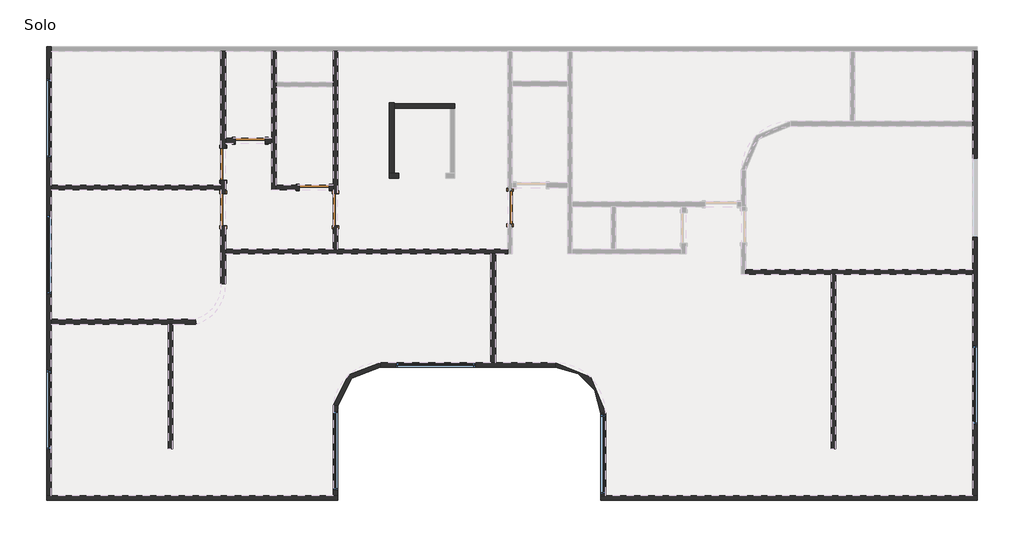
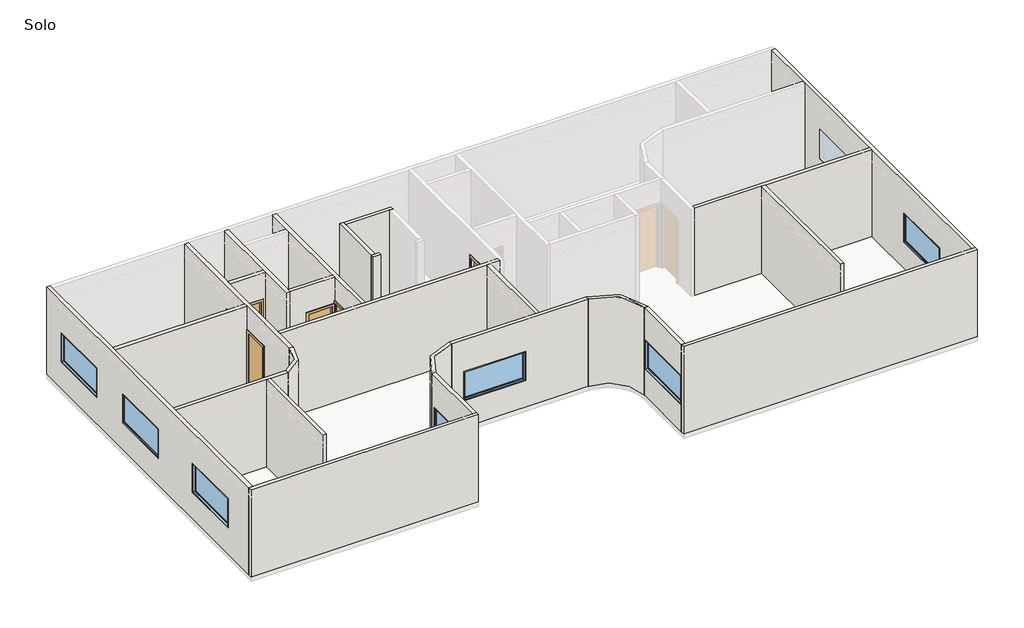
# One storey, part 1 of 2: 25 walls, 7 windows, 6 doors.
"""IFC4 building model written with IfcOpenShell, lengths in millimetres."""

import ifcopenshell
import ifcopenshell.guid

model = None  # the IFC model being written
_history = None  # IfcOwnerHistory: only IFC2X3 demands one
_inside = {}  # id of a spatial element -> (the spatial element, [elements in it])
_under = {}  # id of a project, library or spatial element -> (it, [spatial elements below it])
_declared = {}  # id of a project -> (the project, [libraries it declares])
_typed = {}  # id of a type object -> (the type object, [elements of that type])
_made_of = {}  # id of a material, layer set ... -> (it, [elements and type objects made of it])


def new_model(schema):
    """Start an empty IFC model of exactly this schema.

    Asked for "IFC4X3", IfcOpenShell would pick the latest addendum, in which some entities
    have other attributes; the version numbers below select the first issue.
    IFC2X3 requires an IfcOwnerHistory on every rooted entity: one is made here for all.
    """
    global model, _history
    if schema == "IFC4X3":
        model = ifcopenshell.file(schema_version=(4, 3, 0, 0))
    else:
        model = ifcopenshell.file(schema=schema)
    _inside.clear()
    _under.clear()
    _declared.clear()
    _typed.clear()
    _made_of.clear()
    _history = None
    if model.schema == "IFC2X3":
        org = make("IfcOrganization", Name="unknown")
        user = make(
            "IfcPersonAndOrganization",
            ThePerson=make("IfcPerson", FamilyName="unknown"),
            TheOrganization=org,
        )
        app = make(
            "IfcApplication",
            ApplicationDeveloper=org,
            Version="unknown",
            ApplicationFullName="unknown",
            ApplicationIdentifier="unknown",
        )
        _history = make(
            "IfcOwnerHistory",
            OwningUser=user,
            OwningApplication=app,
            ChangeAction="ADDED",
            CreationDate=0,
        )
    return model


def make(cls, **values):
    """One entity of the class cls with the attributes given. An attribute that is None is left unset."""
    return model.create_entity(
        cls, **{name: value for name, value in values.items() if value is not None}
    )


def rooted(cls, **values):
    """An entity with a GlobalId (a new one), such as an element, a storey or a relation."""
    return make(cls, GlobalId=ifcopenshell.guid.new(), OwnerHistory=_history, **values)


def si_unit(unit_type, name, prefix=None):
    """IfcSIUnit, for example si_unit("LENGTHUNIT", "METRE", prefix="MILLI")."""
    return make("IfcSIUnit", UnitType=unit_type, Prefix=prefix, Name=name)


def assignment(units):
    """IfcUnitAssignment: the units of a project."""
    return None if units is None else make("IfcUnitAssignment", Units=units)


def point(xyz):
    """IfcCartesianPoint."""
    return None if xyz is None else make("IfcCartesianPoint", Coordinates=xyz)


def direction(xyz):
    """IfcDirection."""
    return None if xyz is None else make("IfcDirection", DirectionRatios=xyz)


def frame(location, z_axis=None, x_axis=None):
    """IfcAxis2Placement3D, a coordinate frame: its origin and axes. An axis left out is left unset."""
    return make(
        "IfcAxis2Placement3D",
        Location=point(location),
        Axis=direction(z_axis),
        RefDirection=direction(x_axis),
    )


def frame_2d(location, x_axis=None):
    """IfcAxis2Placement2D, a coordinate frame in the plane: its origin and x axis."""
    return make(
        "IfcAxis2Placement2D", Location=point(location), RefDirection=direction(x_axis)
    )


def origin():
    """The frame at (0, 0, 0) with its axes left unset."""
    return frame((0.0, 0.0, 0.0))


def origin_with_axes():
    """The frame at (0, 0, 0) with the z axis (0, 0, 1) and the x axis (1, 0, 0) written out."""
    return frame((0.0, 0.0, 0.0), z_axis=(0.0, 0.0, 1.0), x_axis=(1.0, 0.0, 0.0))


def place(relative_to, where):
    """IfcLocalPlacement: puts the frame where relative to a parent placement (None: the world)."""
    return make(
        "IfcLocalPlacement", PlacementRelTo=relative_to, RelativePlacement=where
    )


def context(
    kind, dimensions, precision=None, world=None, true_north=None, identifier=None
):
    """IfcGeometricRepresentationContext, for example the 3D "Model" context."""
    return make(
        "IfcGeometricRepresentationContext",
        ContextIdentifier=identifier,
        ContextType=kind,
        CoordinateSpaceDimension=dimensions,
        Precision=precision,
        WorldCoordinateSystem=world,
        TrueNorth=true_north,
    )


def project(units=None, contexts=None):
    """IfcProject with its units and contexts."""
    return rooted(
        "IfcProject",
        Name="project",
        RepresentationContexts=contexts,
        UnitsInContext=assignment(units),
    )


def spatial(cls, under=None, at=None, **own):
    """A site, building, storey or space (cls), placed at a placement, below another one or the project."""
    s = rooted(cls, ObjectPlacement=at, **own)
    if under is not None:
        _under.setdefault(under.id(), (under, []))[1].append(s)
    return s


def polyline(points):
    """IfcPolyline through the points."""
    return make("IfcPolyline", Points=[point(p) for p in points])


def circle_curve(where, radius):
    """IfcCircle in the frame where."""
    return make("IfcCircle", Position=where, Radius=radius)


def trimmed(basis, trim1, trim2, sense, master):
    """IfcTrimmedCurve: the piece of a basis curve between two trims."""
    return make(
        "IfcTrimmedCurve",
        BasisCurve=basis,
        Trim1=trim1,
        Trim2=trim2,
        SenseAgreement=sense,
        MasterRepresentation=master,
    )


def segment(curve, same_sense, transition):
    """IfcCompositeCurveSegment."""
    return make(
        "IfcCompositeCurveSegment",
        Transition=transition,
        SameSense=same_sense,
        ParentCurve=curve,
    )


def composite_curve(segments, self_intersect=None):
    """IfcCompositeCurve: segments joined end to end."""
    return make("IfcCompositeCurve", Segments=segments, SelfIntersect=self_intersect)


def outline(outer, holes=None, kind="AREA"):
    """IfcArbitraryClosedProfileDef: a profile drawn as a closed curve; with holes, ...WithVoids."""
    if holes is None:
        return make("IfcArbitraryClosedProfileDef", ProfileType=kind, OuterCurve=outer)
    return make(
        "IfcArbitraryProfileDefWithVoids",
        ProfileType=kind,
        OuterCurve=outer,
        InnerCurves=holes,
    )


def extrude(swept, where, along, depth):
    """IfcExtrudedAreaSolid: the profile swept, set in the frame where, extruded along a direction by depth."""
    return make(
        "IfcExtrudedAreaSolid",
        SweptArea=swept,
        Position=where,
        ExtrudedDirection=direction(along),
        Depth=depth,
    )


def faces_of(points, faces, orient=None, outer=None):
    """IfcFace entities. A face is a list of loops; a loop is a list of indices into points, from 0.

    orient and outer hold one flag for each loop. By default every Orientation is true, the
    first loop of a face is its IfcFaceOuterBound and the others are IfcFaceBound.
    """
    made = []
    for i, loops in enumerate(faces):
        bounds = []
        for j, loop in enumerate(loops):
            is_outer = j == 0 if outer is None else outer[i][j]
            bounds.append(
                make(
                    "IfcFaceOuterBound" if is_outer else "IfcFaceBound",
                    Bound=make("IfcPolyLoop", Polygon=[points[k] for k in loop]),
                    Orientation=True if orient is None else orient[i][j],
                )
            )
        made.append(make("IfcFace", Bounds=bounds))
    return made


def faceted_brep(points, faces, orient=None, outer=None, voids=None):
    """IfcFacetedBrep: a solid bounded by flat faces; with voids (closed shells), ...WithVoids."""
    shared = [point(p) for p in points]
    hull = make("IfcClosedShell", CfsFaces=faces_of(shared, faces, orient, outer))
    if voids is None:
        return make("IfcFacetedBrep", Outer=hull)
    return make(
        "IfcFacetedBrepWithVoids",
        Outer=hull,
        Voids=[
            make(cls, CfsFaces=faces_of(shared, fs, o, b)) for cls, fs, o, b in voids
        ],
    )


def shape(context_of_items, identifier, shape_type, items):
    """IfcShapeRepresentation: the items that make up one representation, for example the "Body"."""
    return make(
        "IfcShapeRepresentation",
        ContextOfItems=context_of_items,
        RepresentationIdentifier=identifier,
        RepresentationType=shape_type,
        Items=items,
    )


def source(mapping_origin, context_of_items, identifier, shape_type, items):
    """IfcRepresentationMap: a shape defined once, which mapped items show again and again."""
    return make(
        "IfcRepresentationMap",
        MappingOrigin=mapping_origin,
        MappedRepresentation=shape(context_of_items, identifier, shape_type, items),
    )


def transform(
    local_origin,
    x_axis=None,
    y_axis=None,
    z_axis=None,
    scale=None,
    scale2=None,
    scale3=None,
    uniform=True,
):
    """IfcCartesianTransformationOperator3D, or its non-uniform kind. x_axis, y_axis, z_axis: its Axis1, 2, 3."""
    if uniform:
        return make(
            "IfcCartesianTransformationOperator3D",
            Axis1=direction(x_axis),
            Axis2=direction(y_axis),
            LocalOrigin=point(local_origin),
            Scale=scale,
            Axis3=direction(z_axis),
        )
    return make(
        "IfcCartesianTransformationOperator3DnonUniform",
        Axis1=direction(x_axis),
        Axis2=direction(y_axis),
        LocalOrigin=point(local_origin),
        Scale=scale,
        Axis3=direction(z_axis),
        Scale2=scale2,
        Scale3=scale3,
    )


def mapped(mapping_source, mapping_target):
    """IfcMappedItem: shows the shape of a source again, moved by a transform."""
    return make(
        "IfcMappedItem", MappingSource=mapping_source, MappingTarget=mapping_target
    )


def made_of(thing, what):
    """Note that an element or type object is made of a material, layer set ...; save() writes the relation."""
    if what is not None:
        _made_of.setdefault(what.id(), (what, []))[1].append(thing)
    return thing


def element(
    cls,
    number,
    at=None,
    inside=None,
    cuts=None,
    type_object=None,
    material=None,
    context=None,
    identifier="Body",
    shape_type=None,
    held_by="IfcProductDefinitionShape",
    body=None,
    shapes=None,
    **own,
):
    """One element of the class cls, such as IfcWall. Its Tag is "e" and its number.

    at: its placement. inside: the storey or other place that contains it. cuts: it is an
    opening in that element (IfcRelVoidsElement). A single representation is given by context,
    identifier, shape_type and body (its items); several are given by shapes. held_by: the class
    of the entity that holds the representations. save() writes the other relations.
    """
    e = rooted(cls, Tag="e%d" % number, ObjectPlacement=at, **own)
    if body is not None:
        shapes = [shape(context, identifier, shape_type, body)]
    if shapes is not None:
        e.Representation = make(held_by, Representations=shapes)
    if inside is not None:
        _inside.setdefault(inside.id(), (inside, []))[1].append(e)
    if cuts is not None:
        rooted(
            "IfcRelVoidsElement", RelatingBuildingElement=cuts, RelatedOpeningElement=e
        )
    if type_object is not None:
        _typed.setdefault(type_object.id(), (type_object, []))[1].append(e)
    return made_of(e, material)


def aggregate(whole, parts):
    """IfcRelAggregates: a whole, such as a stair, and the parts it consists of."""
    return rooted("IfcRelAggregates", RelatingObject=whole, RelatedObjects=parts)


def save(model, path):
    """Write the relations noted so far, then the file.

    IfcRelAggregates (storeys below a building ...), IfcRelContainedInSpatialStructure (elements
    in a storey), IfcRelDefinesByType, IfcRelAssociatesMaterial and IfcRelDeclares: one each for
    every whole, place, type object, material and project.
    """
    for whole, parts in _under.values():
        aggregate(whole, parts)
    for where, things in _inside.values():
        rooted(
            "IfcRelContainedInSpatialStructure",
            RelatedElements=things,
            RelatingStructure=where,
        )
    for kind, things in _typed.values():
        rooted("IfcRelDefinesByType", RelatedObjects=things, RelatingType=kind)
    for what, things in _made_of.values():
        rooted("IfcRelAssociatesMaterial", RelatedObjects=things, RelatingMaterial=what)
    for by, libraries in _declared.values():
        rooted("IfcRelDeclares", RelatingContext=by, RelatedDefinitions=libraries)
    model.write(path)


def door_0762_x_2032mm_ca16c8eb(model_context):
    return source(origin(), model_context, "Body", "SweptSolid", [
        extrude(outline(polyline([(2108.0, -457.0), (0.0, -457.0), (0.0, -381.0), (2032.0, -381.0), (2032.0, 381.0), (0.0, 381.0), (0.0, 457.0), (2108.0, 457.0), (2108.0, -457.0)])), frame((0.0, 60.0, 0.0), z_axis=(0.0, 1.0, 0.0), x_axis=(0.0, 0.0, 1.0)), (0.0, 0.0, 1.0), 25.0),
        extrude(outline(polyline([(2108.0, 457.0), (2108.0, -457.0), (0.0, -457.0), (0.0, -381.0), (2032.0, -381.0), (2032.0, 381.0), (0.0, 381.0), (0.0, 457.0), (2108.0, 457.0)])), frame((0.0, -85.0, 0.0), z_axis=(0.0, 1.0, 0.0), x_axis=(0.0, 0.0, 1.0)), (0.0, 0.0, 1.0), 25.0),
        extrude(outline(polyline([(381.0, 9.0), (-381.0, 9.0), (-381.0, 60.0), (381.0, 60.0), (381.0, 9.0)])), origin_with_axes(), (0.0, 0.0, 1.0), 2032.0),
    ])


def door_0813_x_2134mm_8eb04c96(model_context):
    return source(origin(), model_context, "Body", "SweptSolid", [
        extrude(outline(polyline([(2210.0, -482.5), (0.0, -482.5), (0.0, -406.5), (2134.0, -406.5), (2134.0, 406.5), (0.0, 406.5), (0.0, 482.5), (2210.0, 482.5), (2210.0, -482.5)])), frame((0.0, -85.0, 0.0), z_axis=(0.0, 1.0, 0.0), x_axis=(0.0, 0.0, 1.0)), (0.0, 0.0, 1.0), 25.0),
        extrude(outline(polyline([(2210.0, 482.5), (2210.0, -482.5), (0.0, -482.5), (0.0, -406.5), (2134.0, -406.5), (2134.0, 406.5), (0.0, 406.5), (0.0, 482.5), (2210.0, 482.5)])), frame((0.0, 60.0, 0.0), z_axis=(0.0, 1.0, 0.0), x_axis=(0.0, 0.0, 1.0)), (0.0, 0.0, 1.0), 25.0),
        extrude(outline(polyline([(406.5, -9.0), (406.5, -60.0), (-406.5, -60.0), (-406.5, -9.0), (406.5, -9.0)])), origin_with_axes(), (0.0, 0.0, 1.0), 2134.0),
    ])


def door_0813_x_2134mm_314d41b2(model_context):
    return source(origin(), model_context, "Body", "SweptSolid", [
        extrude(outline(polyline([(2210.0, -482.5), (0.0, -482.5), (0.0, -406.5), (2134.0, -406.5), (2134.0, 406.5), (0.0, 406.5), (0.0, 482.5), (2210.0, 482.5), (2210.0, -482.5)])), frame((0.0, 60.0, 0.0), z_axis=(0.0, 1.0, 0.0), x_axis=(0.0, 0.0, 1.0)), (0.0, 0.0, 1.0), 25.0),
        extrude(outline(polyline([(2210.0, 482.5), (2210.0, -482.5), (0.0, -482.5), (0.0, -406.5), (2134.0, -406.5), (2134.0, 406.5), (0.0, 406.5), (0.0, 482.5), (2210.0, 482.5)])), frame((0.0, -85.0, 0.0), z_axis=(0.0, 1.0, 0.0), x_axis=(0.0, 0.0, 1.0)), (0.0, 0.0, 1.0), 25.0),
        extrude(outline(polyline([(406.5, 9.0), (-406.5, 9.0), (-406.5, 60.0), (406.5, 60.0), (406.5, 9.0)])), origin_with_axes(), (0.0, 0.0, 1.0), 2134.0),
    ])


def m_fixo_2000_x_1000mm_897e8a61(model_context):
    return source(origin(), model_context, "Body", "SweptSolid", [
        extrude(outline(polyline([(-937.0, 38.0), (937.0, 38.0), (937.0, 26.0), (-937.0, 26.0), (-937.0, 38.0)])), frame((0.0, 0.0, 978.0), z_axis=(0.0, 0.0, 1.0), x_axis=(1.0, 0.0, 0.0)), (0.0, 0.0, 1.0), 874.0),
        extrude(outline(polyline([(1896.0, -981.0), (934.0, -981.0), (934.0, 981.0), (1896.0, 981.0), (1896.0, -981.0)]), holes=[polyline([(1852.0, -937.0), (1852.0, 937.0), (978.0, 937.0), (978.0, -937.0), (1852.0, -937.0)])]), frame((0.0, 10.0, 0.0), z_axis=(0.0, 1.0, 0.0), x_axis=(0.0, 0.0, 1.0)), (0.0, 0.0, 1.0), 44.0),
        extrude(outline(polyline([(1915.0, -1000.0), (915.0, -1000.0), (915.0, 1000.0), (1915.0, 1000.0), (1915.0, -1000.0)]), holes=[polyline([(1896.0, -981.0), (1896.0, 981.0), (934.0, 981.0), (934.0, -981.0), (1896.0, -981.0)])]), frame((0.0, 10.0, 0.0), z_axis=(0.0, 1.0, 0.0), x_axis=(0.0, 0.0, 1.0)), (0.0, 0.0, 1.0), 63.0),
        extrude(outline(polyline([(1915.0, -1000.0), (915.0, -1000.0), (915.0, 1000.0), (1915.0, 1000.0), (1915.0, -1000.0)]), holes=[polyline([(1883.0, -968.0), (1883.0, 968.0), (947.0, 968.0), (947.0, -968.0), (1883.0, -968.0)])]), frame((0.0, -47.0, 0.0), z_axis=(0.0, 1.0, 0.0), x_axis=(0.0, 0.0, 1.0)), (0.0, 0.0, 1.0), 57.0),
    ])


model = new_model("IFC4")

# Units and contexts
model_context = context("Model", 3, world=origin())
ifc_project = project(units=[si_unit("LENGTHUNIT", "METRE", prefix="MILLI")], contexts=[model_context])

# Site, building, storey
site = spatial("IfcSite", under=ifc_project)
building = spatial("IfcBuilding", under=site)
storey = spatial("IfcBuildingStorey", under=building, Name="Solo", Elevation=0.0)

# Doors
placement = place(None, origin())
door_0762_x_2032mm_shape = door_0762_x_2032mm_ca16c8eb(model_context)
element("IfcDoor", 1, ObjectType="M_Folha única : 0762 x 2032mm", at=placement, inside=storey, context=model_context, shape_type="MappedRepresentation", body=[
    mapped(door_0762_x_2032mm_shape, transform((-6942.4242496, 3045.4313177, 0.0), x_axis=(1.0, 0.0, 0.0), y_axis=(0.0, 1.0, 0.0), z_axis=(0.0, 0.0, 1.0))),
])
element("IfcDoor", 2, ObjectType="M_Folha única : 0762 x 2032mm", at=placement, inside=storey, context=model_context, shape_type="MappedRepresentation", body=[
    mapped(door_0762_x_2032mm_shape, transform((-5318.5462561, 1860.3975855, 0.0), x_axis=(1.0, 0.0, 0.0), y_axis=(0.0, 1.0, 0.0), z_axis=(0.0, 0.0, 1.0))),
])
door_0813_x_2134mm_shape = door_0813_x_2134mm_8eb04c96(model_context)
element("IfcDoor", 3, ObjectType="M_Folha única : 0813 x 2134mm", at=placement, inside=storey, context=model_context, shape_type="MappedRepresentation", body=[
    mapped(door_0813_x_2134mm_shape, transform((-7627.5462561, 2452.9144516, 0.0), x_axis=(0.0, -1.0, 0.0), y_axis=(1.0, 0.0, 0.0), z_axis=(0.0, 0.0, 1.0))),
])
element("IfcDoor", 4, ObjectType="M_Folha única : 0813 x 2134mm", at=placement, inside=storey, context=model_context, shape_type="MappedRepresentation", body=[
    mapped(door_0813_x_2134mm_shape, transform((-350.3138992, 1353.4744284, 0.0), x_axis=(0.0, 1.0, 0.0), y_axis=(-1.0, 0.0, 0.0), z_axis=(0.0, 0.0, 1.0))),
])
door_0813_x_2134mm_2_shape = door_0813_x_2134mm_314d41b2(model_context)
element("IfcDoor", 5, ObjectType="M_Folha única : 0813 x 2134mm", at=placement, inside=storey, context=model_context, shape_type="MappedRepresentation", body=[
    mapped(door_0813_x_2134mm_2_shape, transform((-7627.5462561, 1293.8975855, 0.0), x_axis=(0.0, 1.0, 0.0), y_axis=(-1.0, 0.0, 0.0), z_axis=(0.0, 0.0, 1.0))),
])
element("IfcDoor", 6, ObjectType="M_Folha única : 0813 x 2134mm", at=placement, inside=storey, context=model_context, shape_type="MappedRepresentation", body=[
    mapped(door_0813_x_2134mm_2_shape, transform((-4777.5462561, 1293.8975855, 0.0), x_axis=(0.0, 1.0, 0.0), y_axis=(-1.0, 0.0, 0.0), z_axis=(0.0, 0.0, 1.0))),
])

# Walls
element("IfcWall", 7, ObjectType="Genérico - 120 mm - Preenchido 2", at=placement, inside=storey, context=model_context, shape_type="Brep", body=[
    faceted_brep([(-7687.5462561, 2046.4144516, 0.0), (-7687.5462561, 1920.3975855, 0.0), (-7687.5462561, 1800.3975855, 0.0), (-7687.5462561, 1700.3975855, 0.0), (-7687.5462561, 1700.3975855, 2134.0), (-7687.5462561, 887.3975855, 2134.0), (-7687.5462561, 887.3975855, 0.0), (-7687.5462561, -585.6507938, 0.0), (-7687.5462561, -585.6507938, 3000.0), (-7687.5462561, 1800.3975855, 3000.0), (-7687.5462561, 1920.3975855, 3000.0), (-7687.5462561, 5315.4313177, 3000.0), (-7687.5462561, 5315.4313177, 0.0), (-7687.5462561, 2859.4144516, 0.0), (-7687.5462561, 2859.4144516, 2134.0), (-7687.5462561, 2046.4144516, 2134.0), (-7567.5462561, 1700.3975855, 2134.0), (-7567.5462561, 1700.3975855, 0.0), (-7567.5462561, 2046.4144516, 0.0), (-7567.5462561, 2046.4144516, 2134.0), (-7567.5462561, 2859.4144516, 2134.0), (-7567.5462561, 2859.4144516, 0.0), (-7567.5462561, 2985.4313177, 0.0), (-7567.5462561, 3105.4313177, 0.0), (-7567.5462561, 5315.4313177, 0.0), (-7567.5462561, 5315.4313177, 3000.0), (-7567.5462561, 3105.4313177, 3000.0), (-7567.5462561, 2985.4313177, 3000.0), (-7567.5462561, 293.7558339, 3000.0), (-7567.5462561, 173.7558339, 3000.0), (-7567.5462561, -583.5861825, 3000.0), (-7567.5462561, -583.5861825, 0.0), (-7567.5462561, 173.7558339, 0.0), (-7567.5462561, 293.7558339, 0.0), (-7567.5462561, 887.3975855, 0.0), (-7567.5462561, 887.3975855, 2134.0)], [[[0, 1, 2, 3, 4, 5, 6, 7, 8, 9, 10, 11, 12, 13, 14, 15]], [[16, 17, 18, 19, 20, 21, 22, 23, 24, 25, 26, 27, 28, 29, 30, 31, 32, 33, 34, 35]], [[13, 12, 24, 23, 22, 21]], [[18, 17, 3, 2, 1, 0]], [[34, 33, 32, 31, 7, 6]], [[11, 10, 9, 8, 30, 29, 28, 27, 26, 25]], [[12, 11, 25, 24]], [[8, 7, 31, 30]], [[19, 18, 0, 15]], [[20, 19, 15, 14]], [[21, 20, 14, 13]], [[4, 3, 17, 16]], [[5, 4, 16, 35]], [[6, 5, 35, 34]]]),
])
element("IfcWall", 8, ObjectType="Genérico - 120 mm - Preenchido 2", at=placement, inside=storey, context=model_context, shape_type="Brep", body=[
    faceted_brep([(11383.1038545, 5315.4313177, 0.0), (11383.1038545, 3535.4313177, 0.0), (11383.1038545, 3415.4313177, 0.0), (11383.1038545, -220.1148653, 0.0), (11383.1038545, -340.1148653, 0.0), (11383.1038545, -5955.2378912, 0.0), (11383.1038545, -5955.2378912, 3000.0), (11383.1038545, -340.1148653, 3000.0), (11383.1038545, -220.1148653, 3000.0), (11383.1038545, 3415.4313177, 3000.0), (11383.1038545, 3535.4313177, 3000.0), (11383.1038545, 5315.4313177, 3000.0), (11383.1038545, -4147.6763782, 915.0), (11383.1038545, -2147.6763782, 915.0), (11383.1038545, -2147.6763782, 1915.0), (11383.1038545, -4147.6763782, 1915.0), (11383.1038545, 2597.6582262, 915.0), (11383.1038545, 2597.6582262, 1915.0), (11383.1038545, 597.6582262, 1915.0), (11383.1038545, 597.6582262, 915.0), (11503.1038545, 5315.4313177, 0.0), (11503.1038545, 5315.4313177, 3000.0), (11503.1038545, -5955.2378912, 3000.0), (11503.1038545, -5955.2378912, 0.0), (11503.1038545, -4147.6763782, 915.0), (11503.1038545, -4147.6763782, 1915.0), (11503.1038545, -2147.6763782, 1915.0), (11503.1038545, -2147.6763782, 915.0), (11503.1038545, 2597.6582262, 915.0), (11503.1038545, 597.6582262, 915.0), (11503.1038545, 597.6582262, 1915.0), (11503.1038545, 2597.6582262, 1915.0)], [[[0, 1, 2, 3, 4, 5, 6, 7, 8, 9, 10, 11], [12, 13, 14, 15], [16, 17, 18, 19]], [[20, 21, 22, 23], [24, 25, 26, 27], [28, 29, 30, 31]], [[5, 4, 3, 2, 1, 0, 20, 23]], [[11, 10, 9, 8, 7, 6, 22, 21]], [[0, 11, 21, 20]], [[6, 5, 23, 22]], [[25, 24, 12, 15]], [[26, 25, 15, 14]], [[27, 26, 14, 13]], [[24, 27, 13, 12]], [[17, 16, 28, 31]], [[18, 17, 31, 30]], [[19, 18, 30, 29]], [[16, 19, 29, 28]]]),
])
element("IfcWall", 9, ObjectType="Genérico - 120 mm - Preenchido 2", at=placement, inside=storey, context=model_context, shape_type="Brep", body=[
    faceted_brep([(11503.1038545, -5955.2378912, 0.0), (11383.1038545, -5955.2378912, 0.0), (2072.392469, -5955.2378912, 0.0), (1952.392469, -5955.2378912, 0.0), (1952.392469, -5955.2378912, 3000.0), (2072.392469, -5955.2378912, 3000.0), (11383.1038545, -5955.2378912, 3000.0), (11503.1038545, -5955.2378912, 3000.0), (11503.1038545, -6075.2378912, 0.0), (11503.1038545, -6075.2378912, 3000.0), (1952.392469, -6075.2378912, 3000.0), (1952.392469, -6075.2378912, 0.0)], [[[0, 1, 2, 3, 4, 5, 6, 7]], [[8, 9, 10, 11]], [[3, 2, 1, 0, 8, 11]], [[7, 6, 5, 4, 10, 9]], [[4, 3, 11, 10]], [[0, 7, 9, 8]]]),
])
element("IfcWall", 10, ObjectType="Genérico - 120 mm - Preenchido 2", at=placement, inside=storey, context=model_context, shape_type="SweptSolid", body=[
    extrude(outline(polyline([(-5955.2378912, 0.0), (-5955.2378912, 3000.0), (-3863.6287272, 3000.0), (-3863.6287272, 0.0), (-5955.2378912, 0.0)]), holes=[polyline([(-3909.4333092, 915.0), (-3909.4333092, 1915.0), (-5909.4333092, 1915.0), (-5909.4333092, 915.0), (-3909.4333092, 915.0)])]), frame((1952.392469, 0.0, 0.0), z_axis=(1.0, 0.0, 0.0), x_axis=(0.0, 1.0, 0.0)), (0.0, 0.0, 1.0), 120.0),
])
element("IfcWall", 11, ObjectType="Genérico - 120 mm - Preenchido 2", at=placement, inside=storey, context=model_context, shape_type="Brep", body=[
    faceted_brep([(792.392469, -2583.6287272, 0.0), (-717.607531, -2583.6287272, 0.0), (-837.607531, -2583.6287272, 0.0), (-3640.8284375, -2583.6287272, 0.0), (-3640.8284375, -2583.6287272, 3000.0), (-837.607531, -2583.6287272, 3000.0), (-717.607531, -2583.6287272, 3000.0), (792.392469, -2583.6287272, 3000.0), (-3239.2179842, -2583.6287272, 915.0), (-1239.2179842, -2583.6287272, 915.0), (-1239.2179842, -2583.6287272, 1915.0), (-3239.2179842, -2583.6287272, 1915.0), (792.392469, -2703.6287272, 0.0), (792.392469, -2703.6287272, 3000.0), (-3640.8284375, -2703.6287272, 3000.0), (-3640.8284375, -2703.6287272, 0.0), (-3239.2179842, -2703.6287272, 915.0), (-3239.2179842, -2703.6287272, 1915.0), (-1239.2179842, -2703.6287272, 1915.0), (-1239.2179842, -2703.6287272, 915.0)], [[[0, 1, 2, 3, 4, 5, 6, 7], [8, 9, 10, 11]], [[12, 13, 14, 15], [16, 17, 18, 19]], [[3, 2, 1, 0, 12, 15]], [[4, 3, 15, 14]], [[7, 6, 5, 4, 14, 13]], [[0, 7, 13, 12]], [[17, 16, 8, 11]], [[18, 17, 11, 10]], [[19, 18, 10, 9]], [[16, 19, 9, 8]]]),
])
element("IfcWall", 12, ObjectType="Genérico - 120 mm - Preenchido 2", at=placement, inside=storey, context=model_context, shape_type="Brep", body=[
    faceted_brep([(-4719.3676237, -5954.8147341, 0.0), (-4719.3676237, -3673.2373358, 0.0), (-4719.3676237, -3673.2373358, 3000.0), (-4719.3676237, -5954.8147341, 3000.0), (-4719.3676237, -5812.4520359, 915.0), (-4719.3676237, -5812.4520359, 1915.0), (-4719.3676237, -3812.4520359, 1915.0), (-4719.3676237, -3812.4520359, 915.0), (-4839.3676237, -5954.8147341, 0.0), (-4839.3676237, -5954.8147341, 3000.0), (-4839.3676237, -3667.0230345, 3000.0), (-4839.3676237, -3667.0230345, 0.0), (-4839.3676237, -5812.4520359, 915.0), (-4839.3676237, -3812.4520359, 915.0), (-4839.3676237, -3812.4520359, 1915.0), (-4839.3676237, -5812.4520359, 1915.0)], [[[0, 1, 2, 3], [4, 5, 6, 7]], [[8, 9, 10, 11], [12, 13, 14, 15]], [[1, 0, 8, 11]], [[3, 2, 10, 9]], [[2, 1, 11, 10]], [[0, 3, 9, 8]], [[5, 4, 12, 15]], [[6, 5, 15, 14]], [[7, 6, 14, 13]], [[4, 7, 13, 12]]]),
])
element("IfcWall", 13, ObjectType="Genérico - 120 mm - Preenchido 2", at=placement, inside=storey, context=model_context, shape_type="Brep", body=[
    faceted_brep([(-4719.3676237, -5954.8147341, 0.0), (-4839.3676237, -5954.8147341, 0.0), (-11987.7424597, -5954.8147341, 0.0), (-12107.7424597, -5954.8147341, 0.0), (-12107.7424597, -5954.8147341, 3000.0), (-11987.7424597, -5954.8147341, 3000.0), (-4839.3676237, -5954.8147341, 3000.0), (-4719.3676237, -5954.8147341, 3000.0), (-4719.3676237, -6074.8147341, 0.0), (-4719.3676237, -6074.8147341, 3000.0), (-12107.7424597, -6074.8147341, 3000.0), (-12107.7424597, -6074.8147341, 0.0)], [[[0, 1, 2, 3, 4, 5, 6, 7]], [[8, 9, 10, 11]], [[3, 2, 1, 0, 8, 11]], [[7, 6, 5, 4, 10, 9]], [[4, 3, 11, 10]], [[0, 7, 9, 8]]]),
])
element("IfcWall", 14, ObjectType="Genérico - 120 mm - Preenchido 2", at=placement, inside=storey, context=model_context, shape_type="Brep", body=[
    faceted_brep([(-11987.7424597, -5954.8147341, 0.0), (-11987.7424597, -1604.6024145, 0.0), (-11987.7424597, -1484.6024145, 0.0), (-11987.7424597, 1800.3975855, 0.0), (-11987.7424597, 1920.3975855, 0.0), (-11987.7424597, 5315.4313177, 0.0), (-11987.7424597, 5435.4313177, 0.0), (-11987.7424597, 5435.4313177, 3000.0), (-11987.7424597, 5315.4313177, 3000.0), (-11987.7424597, 1920.3975855, 3000.0), (-11987.7424597, 1800.3975855, 3000.0), (-11987.7424597, -1484.6024145, 3000.0), (-11987.7424597, -1604.6024145, 3000.0), (-11987.7424597, -5954.8147341, 3000.0), (-11987.7424597, -2779.7085743, 915.0), (-11987.7424597, -4779.7085743, 915.0), (-11987.7424597, -4779.7085743, 1915.0), (-11987.7424597, -2779.7085743, 1915.0), (-11987.7424597, -842.1024145, 915.0), (-11987.7424597, -842.1024145, 1915.0), (-11987.7424597, 1157.8975855, 1915.0), (-11987.7424597, 1157.8975855, 915.0), (-11987.7424597, 4617.9144516, 915.0), (-11987.7424597, 2617.9144516, 915.0), (-11987.7424597, 2617.9144516, 1915.0), (-11987.7424597, 4617.9144516, 1915.0), (-12107.7424597, -5954.8147341, 0.0), (-12107.7424597, -5954.8147341, 3000.0), (-12107.7424597, 5435.4313177, 3000.0), (-12107.7424597, 5435.4313177, 0.0), (-12107.7424597, -2779.7085743, 915.0), (-12107.7424597, -2779.7085743, 1915.0), (-12107.7424597, -4779.7085743, 1915.0), (-12107.7424597, -4779.7085743, 915.0), (-12107.7424597, -842.1024145, 915.0), (-12107.7424597, 1157.8975855, 915.0), (-12107.7424597, 1157.8975855, 1915.0), (-12107.7424597, -842.1024145, 1915.0), (-12107.7424597, 4617.9144516, 915.0), (-12107.7424597, 4617.9144516, 1915.0), (-12107.7424597, 2617.9144516, 1915.0), (-12107.7424597, 2617.9144516, 915.0)], [[[0, 1, 2, 3, 4, 5, 6, 7, 8, 9, 10, 11, 12, 13], [14, 15, 16, 17], [18, 19, 20, 21], [22, 23, 24, 25]], [[26, 27, 28, 29], [30, 31, 32, 33], [34, 35, 36, 37], [38, 39, 40, 41]], [[6, 5, 4, 3, 2, 1, 0, 26, 29]], [[13, 12, 11, 10, 9, 8, 7, 28, 27]], [[7, 6, 29, 28]], [[0, 13, 27, 26]], [[31, 30, 14, 17]], [[32, 31, 17, 16]], [[33, 32, 16, 15]], [[30, 33, 15, 14]], [[19, 18, 34, 37]], [[20, 19, 37, 36]], [[21, 20, 36, 35]], [[18, 21, 35, 34]], [[39, 38, 22, 25]], [[40, 39, 25, 24]], [[41, 40, 24, 23]], [[38, 41, 23, 22]]]),
])
element("IfcWall", 15, ObjectType="Genérico - 120 mm - Preenchido 2", at=placement, inside=storey, context=model_context, shape_type="Brep", body=[
    faceted_brep([(-6397.5462561, 5315.4313177, 0.0), (-6397.5462561, 3105.4313177, 0.0), (-6397.5462561, 2985.4313177, 0.0), (-6397.5462561, 1800.3975855, 0.0), (-6397.5462561, 1800.3975855, 3000.0), (-6397.5462561, 2985.4313177, 3000.0), (-6397.5462561, 3105.4313177, 3000.0), (-6397.5462561, 5315.4313177, 3000.0), (-6277.5462561, 5315.4313177, 0.0), (-6277.5462561, 5315.4313177, 3000.0), (-6277.5462561, 4529.8633053, 3000.0), (-6277.5462561, 4409.8633053, 3000.0), (-6277.5462561, 1920.3975855, 3000.0), (-6277.5462561, 1800.3975855, 3000.0), (-6277.5462561, 1800.3975855, 0.0), (-6277.5462561, 1920.3975855, 0.0), (-6277.5462561, 4409.8633053, 0.0), (-6277.5462561, 4529.8633053, 0.0)], [[[0, 1, 2, 3, 4, 5, 6, 7]], [[8, 9, 10, 11, 12, 13, 14, 15, 16, 17]], [[3, 2, 1, 0, 8, 17, 16, 15, 14]], [[7, 6, 5, 4, 13, 12, 11, 10, 9]], [[0, 7, 9, 8]], [[4, 3, 14, 13]]]),
])
element("IfcWall", 16, ObjectType="Genérico - 120 mm - Preenchido 2", at=placement, inside=storey, context=model_context, shape_type="SweptSolid", body=[
    extrude(outline(polyline([(2032.0, -6561.4242496), (0.0, -6561.4242496), (0.0, -6397.5462561), (3000.0, -6397.5462561), (3000.0, -7567.5462561), (0.0, -7567.5462561), (0.0, -7323.4242496), (2032.0, -7323.4242496), (2032.0, -6561.4242496)])), frame((0.0, 2985.4313177, 0.0), z_axis=(0.0, 1.0, 0.0), x_axis=(0.0, 0.0, 1.0)), (0.0, 0.0, 1.0), 120.0),
])
element("IfcWall", 17, ObjectType="Genérico - 120 mm - Preenchido 2", at=placement, inside=storey, context=model_context, shape_type="SweptSolid", body=[
    extrude(outline(polyline([(-7687.5462561, 1800.3975855), (-11987.7424597, 1800.3975855), (-11987.7424597, 1920.3975855), (-7687.5462561, 1920.3975855), (-7687.5462561, 1800.3975855)])), origin_with_axes(), (0.0, 0.0, 1.0), 3000.0),
])
element("IfcWall", 18, ObjectType="Genérico - 120 mm - Preenchido 2", at=placement, inside=storey, context=model_context, shape_type="Brep", body=[
    faceted_brep([(-11987.7424597, -1604.6024145, 0.0), (-9023.1250641, -1604.6024145, 0.0), (-8903.1250641, -1604.6024145, 0.0), (-8316.7087575, -1604.6024145, 0.0), (-8316.7087575, -1604.6024145, 3000.0), (-8903.1250641, -1604.6024145, 3000.0), (-9023.1250641, -1604.6024145, 3000.0), (-11987.7424597, -1604.6024145, 3000.0), (-11987.7424597, -1484.6024145, 0.0), (-11987.7424597, -1484.6024145, 3000.0), (-8333.6137775, -1484.6024145, 3000.0), (-8333.6137775, -1484.6024145, 0.0)], [[[0, 1, 2, 3, 4, 5, 6, 7]], [[8, 9, 10, 11]], [[3, 2, 1, 0, 8, 11]], [[7, 6, 5, 4, 10, 9]], [[0, 7, 9, 8]], [[4, 3, 11, 10]]]),
])
element("IfcWall", 19, ObjectType="Genérico - 120 mm - Preenchido 2", at=placement, inside=storey, context=model_context, shape_type="Brep", body=[
    faceted_brep([(-7567.5462561, 173.7558339, 0.0), (-837.607531, 173.7558339, 0.0), (-717.607531, 173.7558339, 0.0), (-410.3138992, 173.7558339, 0.0), (-410.3138992, 173.7558339, 3000.0), (-717.607531, 173.7558339, 3000.0), (-837.607531, 173.7558339, 3000.0), (-7567.5462561, 173.7558339, 3000.0), (-7567.5462561, 293.7558339, 0.0), (-7567.5462561, 293.7558339, 3000.0), (-4837.5462561, 293.7558339, 3000.0), (-4717.5462561, 293.7558339, 3000.0), (-410.3138992, 293.7558339, 3000.0), (-410.3138992, 293.7558339, 0.0), (-4717.5462561, 293.7558339, 0.0), (-4837.5462561, 293.7558339, 0.0)], [[[0, 1, 2, 3, 4, 5, 6, 7]], [[8, 9, 10, 11, 12, 13, 14, 15]], [[3, 2, 1, 0, 8, 15, 14, 13]], [[7, 6, 5, 4, 12, 11, 10, 9]], [[0, 7, 9, 8]], [[4, 3, 13, 12]]]),
])
element("IfcWall", 20, ObjectType="Genérico - 120 mm - Preenchido 2", at=placement, inside=storey, context=model_context, shape_type="SweptSolid", body=[
    extrude(outline(composite_curve([segment(polyline([(-8316.7087575, -1604.6024145), (-8333.6137775, -1484.6024145)]), True, "CONTINUOUS"), segment(trimmed(circle_curve(frame_2d((-8591.3131194, -617.7595428)), 904.3370583), [point((-8333.6137775, -1484.6024145))], [point((-7687.5462561, -585.6507938))], True, "CARTESIAN"), True, "CONTINUOUS"), segment(polyline([(-7687.5462561, -585.6507938), (-7567.5462561, -583.5861825)]), True, "CONTINUOUS"), segment(trimmed(circle_curve(frame_2d((-8591.3131194, -617.7595428)), 1024.3370583), [point((-7567.5462561, -583.5861825))], [point((-8316.7087575, -1604.6024145))], False, "CARTESIAN"), True, "CONTINUOUS")], self_intersect=False)), origin_with_axes(), (0.0, 0.0, 1.0), 3000.0),
])
element("IfcWall", 21, ObjectType="Genérico - 120 mm - Preenchido 2", at=placement, inside=storey, context=model_context, shape_type="SweptSolid", body=[
    extrude(outline(polyline([(-9023.1250641, -4764.547347), (-9023.1250641, -1604.6024145), (-8903.1250641, -1604.6024145), (-8903.1250641, -4764.547347), (-9023.1250641, -4764.547347)])), origin_with_axes(), (0.0, 0.0, 1.0), 3000.0),
])
element("IfcWall", 22, ObjectType="Genérico - 120 mm - Preenchido 2", at=placement, inside=storey, context=model_context, shape_type="SweptSolid", body=[
    extrude(outline(polyline([(-717.607531, 173.7558339), (-717.607531, -2583.6287272), (-837.607531, -2583.6287272), (-837.607531, 173.7558339), (-717.607531, 173.7558339)])), origin_with_axes(), (0.0, 0.0, 1.0), 3000.0),
])
element("IfcWall", 23, ObjectType="Genérico - 120 mm - Preenchido 2", at=placement, inside=storey, context=model_context, shape_type="SweptSolid", body=[
    extrude(outline(composite_curve([segment(polyline([(2072.392469, -3863.6287272), (1952.392469, -3863.6287272)]), True, "CONTINUOUS"), segment(trimmed(circle_curve(frame_2d((792.392469, -3863.6287272)), 1160.0), [point((1952.392469, -3863.6287272))], [point((792.392469, -2703.6287272))], True, "CARTESIAN"), True, "CONTINUOUS"), segment(polyline([(792.392469, -2703.6287272), (792.392469, -2583.6287272)]), True, "CONTINUOUS"), segment(trimmed(circle_curve(frame_2d((792.392469, -3863.6287272)), 1280.0), [point((792.392469, -2583.6287272))], [point((2072.392469, -3863.6287272))], False, "CARTESIAN"), True, "CONTINUOUS")], self_intersect=False)), origin_with_axes(), (0.0, 0.0, 1.0), 3000.0),
])
element("IfcWall", 24, ObjectType="Genérico - 120 mm - Preenchido 2", at=placement, inside=storey, context=model_context, shape_type="SweptSolid", body=[
    extrude(outline(composite_curve([segment(polyline([(-4719.3676237, -3673.2373358), (-4839.3676237, -3667.0230345)]), True, "CONTINUOUS"), segment(trimmed(circle_curve(frame_2d((-3640.8284375, -3788.2857678)), 1204.6579727), [point((-4839.3676237, -3667.0230345))], [point((-3640.8284375, -2583.627795))], False, "CARTESIAN"), True, "CONTINUOUS"), segment(polyline([(-3640.8284375, -2583.627795), (-3640.8284375, -2703.627795)]), True, "CONTINUOUS"), segment(trimmed(circle_curve(frame_2d((-3640.8284375, -3788.2857678)), 1084.6579727), [point((-3640.8284375, -2703.627795))], [point((-4719.3676237, -3673.2373358))], True, "CARTESIAN"), True, "CONTINUOUS")], self_intersect=False)), origin_with_axes(), (0.0, 0.0, 1.0), 3000.0),
])
element("IfcWall", 25, ObjectType="Genérico - 120 mm - Preenchido 2", at=placement, inside=storey, context=model_context, shape_type="Brep", body=[
    faceted_brep([(-4717.5462561, 1700.3975855, 2134.0), (-4717.5462561, 1700.3975855, 0.0), (-4717.5462561, 5315.4313177, 0.0), (-4717.5462561, 5315.4313177, 3000.0), (-4717.5462561, 293.7558339, 3000.0), (-4717.5462561, 293.7558339, 0.0), (-4717.5462561, 887.3975855, 0.0), (-4717.5462561, 887.3975855, 2134.0), (-4837.5462561, 5315.4313177, 0.0), (-4837.5462561, 4529.8633053, 0.0), (-4837.5462561, 4409.8633053, 0.0), (-4837.5462561, 1920.3975855, 0.0), (-4837.5462561, 1800.3975855, 0.0), (-4837.5462561, 1700.3975855, 0.0), (-4837.5462561, 1700.3975855, 2134.0), (-4837.5462561, 887.3975855, 2134.0), (-4837.5462561, 887.3975855, 0.0), (-4837.5462561, 293.7558339, 0.0), (-4837.5462561, 293.7558339, 3000.0), (-4837.5462561, 1800.3975855, 3000.0), (-4837.5462561, 1920.3975855, 3000.0), (-4837.5462561, 4409.8633053, 3000.0), (-4837.5462561, 4529.8633053, 3000.0), (-4837.5462561, 5315.4313177, 3000.0)], [[[0, 1, 2, 3, 4, 5, 6, 7]], [[8, 9, 10, 11, 12, 13, 14, 15, 16, 17, 18, 19, 20, 21, 22, 23]], [[6, 5, 17, 16]], [[2, 1, 13, 12, 11, 10, 9, 8]], [[4, 3, 23, 22, 21, 20, 19, 18]], [[3, 2, 8, 23]], [[5, 4, 18, 17]], [[14, 13, 1, 0]], [[15, 14, 0, 7]], [[16, 15, 7, 6]]]),
])
element("IfcWall", 26, ObjectType="Genérico - 120 mm - Preenchido 2", at=placement, inside=storey, context=model_context, shape_type="SweptSolid", body=[
    extrude(outline(polyline([(2032.0, -4937.5462561), (0.0, -4937.5462561), (0.0, -4837.5462561), (3000.0, -4837.5462561), (3000.0, -6277.5462561), (0.0, -6277.5462561), (0.0, -5699.5462561), (2032.0, -5699.5462561), (2032.0, -4937.5462561)])), frame((0.0, 1800.3975855, 0.0), z_axis=(0.0, 1.0, 0.0), x_axis=(0.0, 0.0, 1.0)), (0.0, 0.0, 1.0), 120.0),
])
element("IfcWall", 27, ObjectType="Genérico - 120 mm - Preenchido 2", at=placement, inside=storey, context=model_context, shape_type="Brep", body=[
    faceted_brep([(-3170.7928649, 2218.2818001, 0.0), (-3289.5233936, 2218.2818001, 0.0), (-3409.5233936, 2218.2818001, 0.0), (-3409.5233936, 2218.2818001, 3000.0), (-3289.5233936, 2218.2818001, 3000.0), (-3170.7928649, 2218.2818001, 3000.0), (-3170.7928649, 2098.2818001, 0.0), (-3170.7928649, 2098.2818001, 3000.0), (-3409.5233936, 2098.2818001, 3000.0), (-3409.5233936, 2098.2818001, 0.0)], [[[0, 1, 2, 3, 4, 5]], [[6, 7, 8, 9]], [[2, 1, 0, 6, 9]], [[5, 4, 3, 8, 7]], [[0, 5, 7, 6]], [[3, 2, 9, 8]]]),
])
element("IfcWall", 28, ObjectType="Genérico - 120 mm - Preenchido 2", at=placement, inside=storey, context=model_context, shape_type="Brep", body=[
    faceted_brep([(-3409.5233936, 4005.1639306, 0.0), (-3409.5233936, 2218.2818001, 0.0), (-3409.5233936, 2218.2818001, 3000.0), (-3409.5233936, 4005.1639306, 3000.0), (-3289.5233936, 4005.1639306, 0.0), (-3289.5233936, 4005.1639306, 3000.0), (-3289.5233936, 3989.8633053, 3000.0), (-3289.5233936, 3869.8633053, 3000.0), (-3289.5233936, 2218.2818001, 3000.0), (-3289.5233936, 2218.2818001, 0.0), (-3289.5233936, 3869.8633053, 0.0), (-3289.5233936, 3989.8633053, 0.0)], [[[0, 1, 2, 3]], [[4, 5, 6, 7, 8, 9, 10, 11]], [[1, 0, 4, 11, 10, 9]], [[3, 2, 8, 7, 6, 5]], [[0, 3, 5, 4]], [[2, 1, 9, 8]]]),
])
element("IfcWall", 29, ObjectType="Genérico - 120 mm - Preenchido 2", at=placement, inside=storey, context=model_context, shape_type="Brep", body=[
    faceted_brep([(-3289.5233936, 3869.8633053, 0.0), (-1870.3138992, 3869.8633053, 0.0), (-1750.3138992, 3869.8633053, 0.0), (-1749.5233936, 3869.8633053, 0.0), (-1749.5233936, 3869.8633053, 3000.0), (-1750.3138992, 3869.8633053, 3000.0), (-1870.3138992, 3869.8633053, 3000.0), (-3289.5233936, 3869.8633053, 3000.0), (-3289.5233936, 3989.8633053, 0.0), (-3289.5233936, 3989.8633053, 3000.0), (-1749.5233936, 3989.8633053, 3000.0), (-1749.5233936, 3989.8633053, 0.0)], [[[0, 1, 2, 3, 4, 5, 6, 7]], [[8, 9, 10, 11]], [[3, 2, 1, 0, 8, 11]], [[4, 3, 11, 10]], [[7, 6, 5, 4, 10, 9]], [[0, 7, 9, 8]]]),
])
element("IfcWall", 30, ObjectType="Genérico - 120 mm - Preenchido 2", at=placement, inside=storey, context=model_context, shape_type="Brep", body=[
    faceted_brep([(11383.1038545, -220.1148653, 0.0), (5632.4537439, -220.1148653, 0.0), (5632.4537439, -220.1148653, 3000.0), (11383.1038545, -220.1148653, 3000.0), (11383.1038545, -340.1148653, 0.0), (11383.1038545, -340.1148653, 3000.0), (7912.4537439, -340.1148653, 3000.0), (7792.4537439, -340.1148653, 3000.0), (5632.4537439, -340.1148653, 3000.0), (5632.4537439, -340.1148653, 0.0), (7792.4537439, -340.1148653, 0.0), (7912.4537439, -340.1148653, 0.0)], [[[0, 1, 2, 3]], [[4, 5, 6, 7, 8, 9, 10, 11]], [[1, 0, 4, 11, 10, 9]], [[3, 2, 8, 7, 6, 5]], [[2, 1, 9, 8]], [[0, 3, 5, 4]]]),
])
element("IfcWall", 31, ObjectType="Genérico - 120 mm - Preenchido 2", at=placement, inside=storey, context=model_context, shape_type="SweptSolid", body=[
    extrude(outline(polyline([(7792.4537439, -4764.547347), (7792.4537439, -340.1148653), (7912.4537439, -340.1148653), (7912.4537439, -4764.547347), (7792.4537439, -4764.547347)])), origin_with_axes(), (0.0, 0.0, 1.0), 3000.0),
])

# Windows
m_fixo_2000_x_1000mm_shape = m_fixo_2000_x_1000mm_897e8a61(model_context)
element("IfcWindow", 32, ObjectType="M_Fixo : 2000 x 1000mm", at=placement, inside=storey, context=model_context, shape_type="MappedRepresentation", body=[
    mapped(m_fixo_2000_x_1000mm_shape, transform((11456.1038545, -3147.6763782, 0.0), x_axis=(0.0, 1.0, 0.0), y_axis=(-1.0, 0.0, 0.0), z_axis=(0.0, 0.0, 1.0))),
])
element("IfcWindow", 33, ObjectType="M_Fixo : 2000 x 1000mm", at=placement, inside=storey, context=model_context, shape_type="MappedRepresentation", body=[
    mapped(m_fixo_2000_x_1000mm_shape, transform((1999.392469, -4909.4333092, 0.0), x_axis=(0.0, -1.0, 0.0), y_axis=(1.0, 0.0, 0.0), z_axis=(0.0, 0.0, 1.0))),
])
element("IfcWindow", 34, ObjectType="M_Fixo : 2000 x 1000mm", at=placement, inside=storey, context=model_context, shape_type="MappedRepresentation", body=[
    mapped(m_fixo_2000_x_1000mm_shape, transform((-4766.3676237, -4812.4520359, 0.0), x_axis=(0.0, 1.0, 0.0), y_axis=(-1.0, 0.0, 0.0), z_axis=(0.0, 0.0, 1.0))),
])
element("IfcWindow", 35, ObjectType="M_Fixo : 2000 x 1000mm", at=placement, inside=storey, context=model_context, shape_type="MappedRepresentation", body=[
    mapped(m_fixo_2000_x_1000mm_shape, transform((-2239.2179842, -2656.6287272, 0.0), x_axis=(1.0, 0.0, 0.0), y_axis=(0.0, 1.0, 0.0), z_axis=(0.0, 0.0, 1.0))),
])
element("IfcWindow", 36, ObjectType="M_Fixo : 2000 x 1000mm", at=placement, inside=storey, context=model_context, shape_type="MappedRepresentation", body=[
    mapped(m_fixo_2000_x_1000mm_shape, transform((-12060.7424597, -3779.7085743, 0.0), x_axis=(0.0, -1.0, 0.0), y_axis=(1.0, 0.0, 0.0), z_axis=(0.0, 0.0, 1.0))),
])
element("IfcWindow", 37, ObjectType="M_Fixo : 2000 x 1000mm", at=placement, inside=storey, context=model_context, shape_type="MappedRepresentation", body=[
    mapped(m_fixo_2000_x_1000mm_shape, transform((-12034.7424597, 157.8975855, 0.0), x_axis=(0.0, 1.0, 0.0), y_axis=(-1.0, 0.0, 0.0), z_axis=(0.0, 0.0, 1.0))),
])
element("IfcWindow", 38, ObjectType="M_Fixo : 2000 x 1000mm", at=placement, inside=storey, context=model_context, shape_type="MappedRepresentation", body=[
    mapped(m_fixo_2000_x_1000mm_shape, transform((-12060.7424597, 3617.9144516, 0.0), x_axis=(0.0, -1.0, 0.0), y_axis=(1.0, 0.0, 0.0), z_axis=(0.0, 0.0, 1.0))),
])

save(model, "model.ifc")

# Revit data of these elements
# Project information
#   Data de emissão do projeto = "Data de emissão"
#   Status do projeto = "Status do projeto"
#   Nome do cliente = "Proprietário"
#   Endereço do projeto = "Insira aqui o endereço"
#   Nome do projeto = "Nome do projeto"
#   Número do projeto = "0001"
# Type "M_Folha única : 0762 x 2032mm"
#   Type Mark = "28"
#   Construction Type Id = "MDOOR"
#   Analytic Construction = "Metal"
#   Thickness = 0.051 m
#   Thermal Resistance (R) = 0.270117 (m²·K)/W
#   Heat Transfer Coefficient (U) = 3.7021 W/(m²·K)
#   Height = 2.032 m
#   Projeção da apara externa = 0.025 m
#   Projeção da apara interna = 0.025 m
#   Largura da apara = 0.076 m
#   Width = 0.762 m
#   Define Thermal Properties by = 1
#   Define Thermal Properties by = 1
#   Material da porta = Porta - Painel
#   Material da moldura = Porta - Batente
#   Visual Light Transmittance = 0
#   Solar Heat Gain Coefficient = 0
#   Function = (empty or 0)
#   Wall Closure = (empty or 0)
# Type "M_Folha única : 0813 x 2134mm"
#   Type Mark = "24"
#   Construction Type Id = "MDOOR"
#   Analytic Construction = "Metal"
#   Thickness = 0.051 m
#   Thermal Resistance (R) = 0.270117 (m²·K)/W
#   Heat Transfer Coefficient (U) = 3.7021 W/(m²·K)
#   Height = 2.134 m
#   Projeção da apara externa = 0.025 m
#   Projeção da apara interna = 0.025 m
#   Largura da apara = 0.076 m
#   Width = 0.813 m
#   Define Thermal Properties by = 1
#   Define Thermal Properties by = 1
#   Material da porta = Porta - Painel
#   Material da moldura = Porta - Batente
#   Visual Light Transmittance = 0
#   Solar Heat Gain Coefficient = 0
#   Function = (empty or 0)
#   Wall Closure = (empty or 0)
# Type "Genérico - 120 mm - Preenchido 2"
#   Layers, outside or top first: 0.12 m no material (function 1)
# Type "M_Fixo : 2000 x 1000mm"
#   Type Mark = "19"
#   Construction Type Id = "GSP4R"
#   Analytic Construction = "Vidraça única Pilkington 1/8 pol"
#   Visual Light Transmittance = 0.9
#   Thermal Resistance (R) = 0.271106 (m²·K)/W
#   Solar Heat Gain Coefficient = 0.78
#   Heat Transfer Coefficient (U) = 3.6886 W/(m²·K)
#   Height = 1.00 m
#   Altura-padrão do peitoril = 0.915 m
#   Width = 2.00 m
#   Janela aplicada = 0.019 m
#   Define Thermal Properties by = 1
#   Material da estrutura externa = Caixilho
#   Material da estrutura interna = Caixilho
#   Material do painel de vidro = Vidro
#   Caixilho = Caixilho
#   Wall Closure = (empty or 0)
# Elements 1, 2 (IfcDoor, "M_Folha única : 0762 x 2032mm")
#   Phase Created = Construção nova
#   Materials on its faces: "Porta - Batente", "Porta - Painel"
# Elements 3, 4, 5, 6 (IfcDoor, "M_Folha única : 0813 x 2134mm")
#   Phase Created = Construção nova
#   Materials on its faces: "Porta - Batente", "Porta - Painel"
# Elements 7, 8, 9, 10, 11, 12, 13, 14, 15, 16, 17, 18, 19, 21, 22, 25, 26, 27, 28, 29, 30, 31 (IfcWall, "Genérico - 120 mm - Preenchido 2")
#   Top Offset = 0.00 m
#   Base Offset = 0.00 m
#   Unconnected Height = 3.00 m
#   wall height = 3.00 m
#   Phase Created = Construção nova
#   Base Constraint = Solo
#   Materials on its faces: "Material pré-definido de parede"
# Elements 20, 23, 24 (IfcWall, "Genérico - 120 mm - Preenchido 2")
#   Top Offset = 0.00 m
#   Base Offset = 0.00 m
#   Unconnected Height = 3.00 m
#   wall height = 3.00 m
#   Phase Created = Construção nova
#   Materials on its faces: "Material pré-definido de parede"
# Element 32 (IfcWindow, "M_Fixo : 2000 x 1000mm")
#   Mark = "1"
#   Phase Created = Construção nova
#   Materials on its faces: "Caixilho", "Vidro"
# Element 33 (IfcWindow, "M_Fixo : 2000 x 1000mm")
#   Mark = "3"
#   Phase Created = Construção nova
#   Materials on its faces: "Caixilho", "Vidro"
# Element 34 (IfcWindow, "M_Fixo : 2000 x 1000mm")
#   Mark = "4"
#   Phase Created = Construção nova
#   Materials on its faces: "Caixilho", "Vidro"
# Element 35 (IfcWindow, "M_Fixo : 2000 x 1000mm")
#   Mark = "5"
#   Phase Created = Construção nova
#   Materials on its faces: "Caixilho", "Vidro"
# Element 36 (IfcWindow, "M_Fixo : 2000 x 1000mm")
#   Mark = "6"
#   Phase Created = Construção nova
#   Materials on its faces: "Caixilho", "Vidro"
# Element 37 (IfcWindow, "M_Fixo : 2000 x 1000mm")
#   Mark = "7"
#   Phase Created = Construção nova
#   Materials on its faces: "Caixilho", "Vidro"
# Element 38 (IfcWindow, "M_Fixo : 2000 x 1000mm")
#   Mark = "8"
#   Phase Created = Construção nova
#   Materials on its faces: "Caixilho", "Vidro"
# Materials
#   "Porta - Painel": class "Madeira", colour RGB 210 159 95, transparency 0, Cost = 0
#   "Porta - Batente": class "Diversos", colour RGB 118 70 51, transparency 0, Cost = 0
#   "Caixilho": class "Madeira", colour RGB 224 178 126, transparency 0, Cost = 0
#   "Vidro": class "Vidro", colour RGB 0 128 192, transparency 0.9, Description = "Vidro de sílica", Cost = 0
#   "Material pré-definido de parede": class "Diversos", colour RGB 128 128 128, transparency 0, Cost = 0
